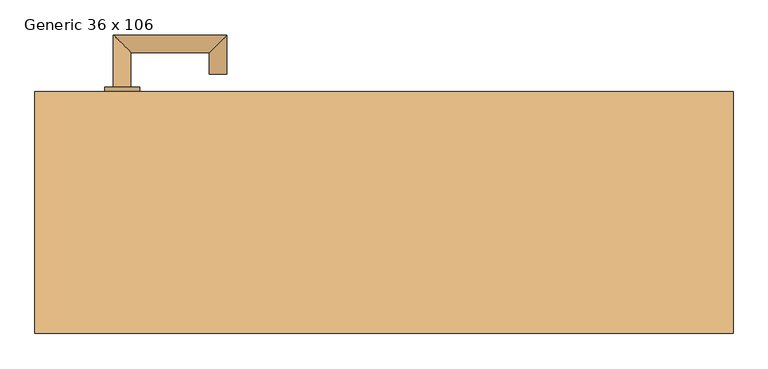
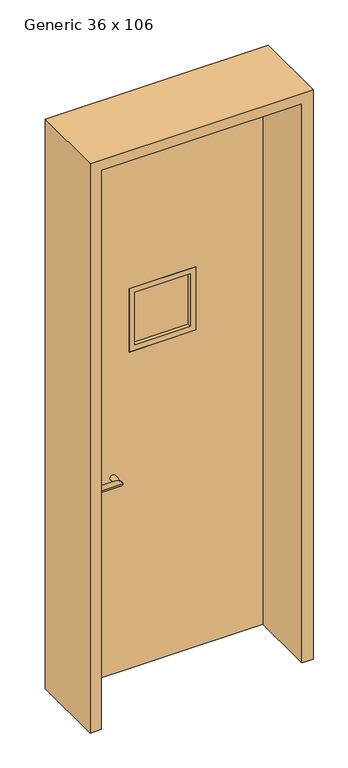
"""IFC4 building model written with IfcOpenShell, lengths in millimetres: door geometry, V_SingleFlush_HOK_I : Generic 36 x 106."""

from ifc_helpers import new_model, si_unit, point, frame, frame_2d, origin, place, context, project, spatial, polyline, circle_curve, ellipse_curve, trimmed, segment, composite_curve, outline, extrude, source, transform, mapped, element, save
from ifc_brep_helpers import plane_surface, cylinder_surface, advanced_brep


def generic_36_x_106_78535582(model_context):
    return source(origin(), model_context, "Body", "SolidModel", [
        advanced_brep(
        [(-393.7, 182.5625, 965.2), (-368.3, 182.5625, 965.2), (-368.3, 233.3625, 965.2), (-393.7, 258.7625, 965.2), (-254.0, 233.3625, 965.2), (-228.6, 258.7625, 965.2), (-228.6, 201.6125, 965.2), (-254.0, 201.6125, 965.2)],
        [
            (0, 1, circle_curve(frame((-381.0, 182.5625, 965.2), z_axis=(0.0, -1.0, 0.0), x_axis=(1.0, 0.0, 0.0)), 12.7)),
            (1, 0, circle_curve(frame((-381.0, 182.5625, 965.2), z_axis=(0.0, -1.0, 0.0), x_axis=(1.0, 0.0, 0.0)), 12.7)),
            (1, 2),
            (2, 3, ellipse_curve(frame((-381.0, 246.0625, 965.2), z_axis=(-0.7071067811867366, -0.7071067811863584, 0.0), x_axis=(0.7071067811863585, -0.7071067811867366, 0.0)), 17.9605122, 12.7)),
            (3, 0),
            (3, 2, ellipse_curve(frame((-381.0, 246.0625, 965.2), z_axis=(-0.7071067811867366, -0.7071067811863584, 0.0), x_axis=(0.7071067811863585, -0.7071067811867366, 0.0)), 17.9605122, 12.7)),
            (2, 4),
            (4, 5, ellipse_curve(frame((-241.3, 246.0625, 965.2), z_axis=(-0.7071067811863584, 0.7071067811867366, 0.0), x_axis=(-0.7071067811867366, -0.7071067811863585, 0.0)), 17.9605122, 12.7)),
            (5, 3),
            (5, 4, ellipse_curve(frame((-241.3, 246.0625, 965.2), z_axis=(-0.7071067811863584, 0.7071067811867366, 0.0), x_axis=(-0.7071067811867366, -0.7071067811863585, 0.0)), 17.9605122, 12.7)),
            (6, 7, circle_curve(frame((-241.3, 201.6125, 965.2), z_axis=(0.0, -1.0, 0.0), x_axis=(-1.0, 0.0, 0.0)), 12.7)),
            (7, 6, circle_curve(frame((-241.3, 201.6125, 965.2), z_axis=(0.0, -1.0, 0.0), x_axis=(-1.0, 0.0, 0.0)), 12.7)),
            (4, 7),
            (6, 5),
        ],
        [
            plane_surface(frame((-381.0, 182.5625, 965.2), z_axis=(0.0, -1.0, 0.0), x_axis=(0.0, 0.0, 1.0))),
            cylinder_surface(frame((-381.0, 182.5625, 965.2), z_axis=(0.0, -1.0, 0.0), x_axis=(1.0, 0.0, 0.0)), 12.7),
            cylinder_surface(frame((-381.0, 246.0625, 965.2), z_axis=(-1.0, 0.0, 0.0), x_axis=(0.0, -1.0, 0.0)), 12.7),
            plane_surface(frame((-241.3, 201.6125, 965.2), z_axis=(0.0, -1.0, 0.0), x_axis=(0.0, 0.0, 1.0))),
            cylinder_surface(frame((-241.3, 246.0625, 965.2), z_axis=(0.0, 1.0, 0.0), x_axis=(-1.0, 0.0, 0.0)), 12.7),
        ],
        [
            (0, [[1, 2]]),
            (1, [[3, 4, 5, -2]]),
            (1, [[-5, 6, -3, -1]]),
            (2, [[7, 8, 9, -4]]),
            (2, [[-9, 10, -7, -6]]),
            (3, [[11, 12]]),
            (4, [[13, -11, 14, -8]]),
            (4, [[-14, -12, -13, -10]]),
        ],
    ),
        extrude(outline(composite_curve([segment(trimmed(circle_curve(frame_2d((965.2, -381.0)), 25.4), [point((965.2, -406.4))], [point((965.2, -355.6))], False, "CARTESIAN"), True, "CONTINUOUS"), segment(trimmed(circle_curve(frame_2d((965.2, -381.0)), 25.4), [point((965.2, -355.6))], [point((965.2, -406.4))], False, "CARTESIAN"), True, "CONTINUOUS")], self_intersect=False)), frame((0.0, 176.2125, 0.0), z_axis=(0.0, 1.0, 0.0), x_axis=(0.0, 0.0, 1.0)), (0.0, 0.0, 1.0), 6.35),
        advanced_brep(
        [(-393.7, 125.4125, 965.2), (-368.3, 125.4125, 965.2), (-393.7, 49.2125, 965.2), (-368.3, 74.6125, 965.2), (-228.6, 49.2125, 965.2), (-254.0, 74.6125, 965.2), (-228.6, 106.3625, 965.2), (-254.0, 106.3625, 965.2)],
        [
            (0, 1, circle_curve(frame((-381.0, 125.4125, 965.2), z_axis=(0.0, 1.0, 0.0), x_axis=(1.0, 0.0, 0.0)), 12.7)),
            (1, 0, circle_curve(frame((-381.0, 125.4125, 965.2), z_axis=(0.0, 1.0, 0.0), x_axis=(1.0, 0.0, 0.0)), 12.7)),
            (0, 2),
            (2, 3, ellipse_curve(frame((-381.0, 61.9125, 965.2), z_axis=(-0.7071067811867366, 0.7071067811863584, 0.0), x_axis=(0.7071067811863585, 0.7071067811867366, 0.0)), 17.9605122, 12.7)),
            (3, 1),
            (3, 2, ellipse_curve(frame((-381.0, 61.9125, 965.2), z_axis=(-0.7071067811867366, 0.7071067811863584, 0.0), x_axis=(0.7071067811863585, 0.7071067811867366, 0.0)), 17.9605122, 12.7)),
            (2, 4),
            (4, 5, ellipse_curve(frame((-241.3, 61.9125, 965.2), z_axis=(-0.7071067811863584, -0.7071067811867366, 0.0), x_axis=(-0.7071067811867366, 0.7071067811863585, 0.0)), 17.9605122, 12.7)),
            (5, 3),
            (5, 4, ellipse_curve(frame((-241.3, 61.9125, 965.2), z_axis=(-0.7071067811863584, -0.7071067811867366, 0.0), x_axis=(-0.7071067811867366, 0.7071067811863585, 0.0)), 17.9605122, 12.7)),
            (6, 7, circle_curve(frame((-241.3, 106.3625, 965.2), z_axis=(0.0, 1.0, 0.0), x_axis=(-1.0, 0.0, 0.0)), 12.7)),
            (7, 6, circle_curve(frame((-241.3, 106.3625, 965.2), z_axis=(0.0, 1.0, 0.0), x_axis=(-1.0, 0.0, 0.0)), 12.7)),
            (4, 6),
            (7, 5),
        ],
        [
            plane_surface(frame((-381.0, 125.4125, 965.2), z_axis=(0.0, 1.0, 0.0), x_axis=(0.0, 0.0, 1.0))),
            cylinder_surface(frame((-381.0, 125.4125, 965.2), z_axis=(0.0, 1.0, 0.0), x_axis=(1.0, 0.0, 0.0)), 12.7),
            cylinder_surface(frame((-381.0, 61.9125, 965.2), z_axis=(-1.0, 0.0, 0.0), x_axis=(0.0, 1.0, 0.0)), 12.7),
            plane_surface(frame((-241.3, 106.3625, 965.2), z_axis=(0.0, 1.0, 0.0), x_axis=(0.0, 0.0, 1.0))),
            cylinder_surface(frame((-241.3, 61.9125, 965.2), z_axis=(0.0, -1.0, 0.0), x_axis=(-1.0, 0.0, 0.0)), 12.7),
        ],
        [
            (0, [[1, 2]]),
            (1, [[-1, 3, 4, 5]]),
            (1, [[-2, -5, 6, -3]]),
            (2, [[-4, 7, 8, 9]]),
            (2, [[-6, -9, 10, -7]]),
            (3, [[11, 12]]),
            (4, [[-8, 13, -12, 14]]),
            (4, [[-10, -14, -11, -13]]),
        ],
    ),
        extrude(outline(composite_curve([segment(trimmed(circle_curve(frame_2d((965.2, -381.0)), 25.4), [point((965.2, -406.4))], [point((965.2, -355.6))], False, "CARTESIAN"), True, "CONTINUOUS"), segment(trimmed(circle_curve(frame_2d((965.2, -381.0)), 25.4), [point((965.2, -355.6))], [point((965.2, -406.4))], False, "CARTESIAN"), True, "CONTINUOUS")], self_intersect=False)), frame((0.0, 125.4125, 0.0), z_axis=(0.0, 1.0, 0.0), x_axis=(0.0, 0.0, 1.0)), (0.0, 0.0, 1.0), 6.35),
        extrude(outline(polyline([(127.0, 150.8125), (-127.0, 150.8125), (-127.0, 157.1625), (127.0, 157.1625), (127.0, 150.8125)])), frame((0.0, 0.0, 1549.4), z_axis=(0.0, 0.0, 1.0), x_axis=(1.0, 0.0, 0.0)), (0.0, 0.0, 1.0), 254.0),
        extrude(outline(polyline([(1828.8, 152.4), (1828.8, -152.4), (1524.0, -152.4), (1524.0, 152.4), (1828.8, 152.4)]), holes=[polyline([(1803.4, 127.0), (1549.4, 127.0), (1549.4, -127.0), (1803.4, -127.0), (1803.4, 127.0)])]), frame((0.0, 131.7625, 0.0), z_axis=(0.0, 1.0, 0.0), x_axis=(0.0, 0.0, 1.0)), (0.0, 0.0, 1.0), 44.45),
        extrude(outline(polyline([(2692.4, -457.2), (0.0, -457.2), (0.0, 457.2), (2692.4, 457.2), (2692.4, -457.2)]), holes=[polyline([(1828.8, 152.4), (1524.0, 152.4), (1524.0, -152.4), (1828.8, -152.4), (1828.8, 152.4)])]), frame((0.0, 131.7625, 0.0), z_axis=(0.0, 1.0, 0.0), x_axis=(0.0, 0.0, 1.0)), (0.0, 0.0, 1.0), 44.45),
        extrude(outline(polyline([(2743.2, 508.0), (2743.2, -508.0), (0.0, -508.0), (0.0, -457.2), (2692.4, -457.2), (2692.4, 457.2), (0.0, 457.2), (0.0, 508.0), (2743.2, 508.0)])), frame((0.0, -176.2125, 0.0), z_axis=(0.0, 1.0, 0.0), x_axis=(0.0, 0.0, 1.0)), (0.0, 0.0, 1.0), 352.425),
    ])


if __name__ == "__main__":
    model = new_model("IFC4")
    model_context = context("Model", 3, world=origin())
    ifc_project = project(units=[si_unit("LENGTHUNIT", "METRE", prefix="MILLI")], contexts=[model_context])
    site = spatial("IfcSite", under=ifc_project)
    building = spatial("IfcBuilding", under=site)
    placement = place(None, origin())
    generic_36_x_106_shape = generic_36_x_106_78535582(model_context)
    element("IfcDoor", 1, ObjectType="V_SingleFlush_HOK_I : Generic 36 x 106", at=placement, inside=building, context=model_context, shape_type="MappedRepresentation", body=[
        mapped(generic_36_x_106_shape, transform((0.0, 0.0, 0.0), x_axis=(1.0, 0.0, 0.0), y_axis=(0.0, 1.0, 0.0), z_axis=(0.0, 0.0, 1.0))),
    ])
    save(model, "model.ifc")

# Revit data of these elements
# Type "V_SingleFlush_HOK_I : Generic 36 x 106"
#   Type Mark = "23"
#   URL_BPD = "http://www.knowledgenet.hok.com/v6/HOK.App.Knet.Web/BPDDetail.aspx?UUID=a7282016-f650-cf84-99e3-8cf7c5ef63ab&Mode=User&ObjectType=2"
#   Manufacturer = "BPD LIBRARY"
#   Equipment = ""
#   DoorTypeMark = ""
#   DoorTypeDescription = ""
#   DoorTagRemark [instance default] = ""
#   DoorPanelType = "V"
#   DoorPanelMaterial = ""
#   DoorPanelGlassType = "GL-02"
#   DoorOpeningIdentifier = ""
#   DoorFrameType = "01"
#   DoorFrameMaterial = ""
#   BIM_ID = ""
#   Assembly Code = "C1020"
#   DoorSwingArc = 90.00°
#   DoorRoughWidth = 3' - 4"
#   DoorRoughHeight = 9' - 0"
#   DoorPanelWidth1 = 3' - 0"
#   DoorPanelThickness = 0' - 1 3/4"
#   DoorPanelHeight = 8' - 10"
#   DoorGlazingWidth = 0' - 10"
#   DoorGlazingMountingHeight = 5' - 1"
#   DoorGlazingHeight = 0' - 10"
#   DoorGlazingFrameWidth = 0' - 1"
#   DoorFrameJambThickness = 0' - 2"
#   DoorFrameHeadThickness = 0' - 2"
#   DoorPanelMaskingRegionVisibility = yes
#   RenderDoorPanel = Door - Panel - Generic
#   RenderDoorGlass = Door - Glazing - Generic
#   RenderDoorFrame = Door - Frame - Generic
#   URL = ""
#   Type Comments = ""
#   Rough Width = 0
#   Rough Height = 0
#   Model = ""
#   Function = (empty or 0)
#   Height = 0
#   Wall Closure = (empty or 0)
#   Width = 0
#   Fire Rating = ""
#   Description = (empty or 0)
#   Cost = 0
# Element 1 (IfcDoor, "V_SingleFlush_HOK_I : Generic 36 x 106")
#   Materials on its faces: "Door - Hardware - Generic", "Door - Panel - Generic", "Door - Frame - Generic", "Door - Glazing - Generic"
# Materials
#   "Door - Panel - Generic": class "Unassigned", colour RGB 196 146 67, transparency 0, Comments = "Rendering appearance not upgraded "
#   "Door - Glazing - Generic": class "Unassigned", colour RGB 0 128 192, transparency 0.75
#   "Door - Frame - Generic": class "Unassigned", colour RGB 164 185 197, transparency 0, Comments = "Rendering appearance not upgraded "
#   "Door - Hardware - Generic": class "Unassigned", colour RGB 164 185 197, transparency 0, Comments = "Rendering appearance not upgraded "
